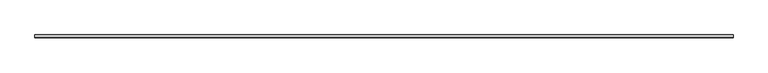
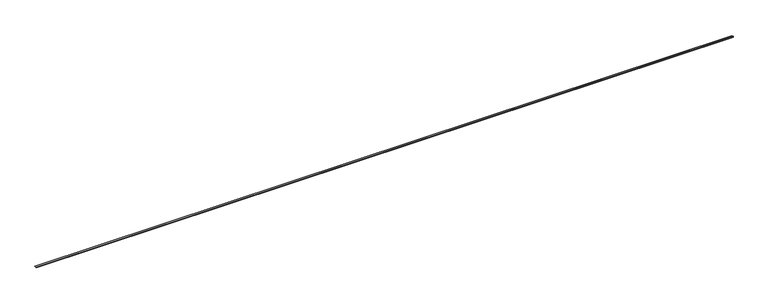
"""IFC4 building model written with IfcOpenShell, lengths in millimetres: proxy geometry, Generic Models 7:Generic Models 1:6:Generic Models 1:6 : Generic Models 7:Generic Models 1:337419:19 : Generic Models 7:Generic Models 1:6:Generic Models 1:6 : Generic Models 7:Generic Models 1:337419:312901."""

from ifc_helpers import new_model, si_unit, frame, origin, place, context, project, spatial, polyline, outline, extrude, source, transform, mapped, element, save


def generic_models_74043bfa(model_context):
    return source(origin(), model_context, "Body", "SweptSolid", [
        extrude(outline(polyline([(-578453.7976341, -216.69375), (-578453.7976341, -218.28125), (-578885.5976341, -218.28125), (-578885.5976341, -97.507466), (-578884.0101341, -97.507466), (-578884.0101341, -216.69375), (-578453.7976341, -216.69375)])), frame((557771.6867239, 0.0, 0.0), z_axis=(1.0, 0.0, 0.0), x_axis=(0.0, 1.0, 0.0)), (0.0, 0.0, 1.0), 109559.725),
    ])


if __name__ == "__main__":
    model = new_model("IFC4")
    model_context = context("Model", 3, world=origin())
    ifc_project = project(units=[si_unit("LENGTHUNIT", "METRE", prefix="MILLI")], contexts=[model_context])
    site = spatial("IfcSite", under=ifc_project)
    building = spatial("IfcBuilding", under=site)
    placement = place(None, origin())
    generic_models_shape = generic_models_74043bfa(model_context)
    element("IfcBuildingElementProxy", 1, Name="Generic Models 7:Generic Models 1:6:Generic Models 1:6 : Generic Models 7:Generic Models 1:337419:19 : Generic Models 7:Generic Models 1:6:Generic Models 1:6 : Generic Models 7:Generic Models 1:337419:312901", ObjectType="Generic Models 7:Generic Models 1:6:Generic Models 1:6 : Generic Models 7:Generic Models 1:337419:19 : Generic Models 7:Generic Models 1:6:Generic Models 1:6 : Generic Models 7:Generic Models 1:337419:312901", at=placement, inside=building, context=model_context, shape_type="MappedRepresentation", body=[
        mapped(generic_models_shape, transform((0.0, 0.0, 0.0), x_axis=(1.0, 0.0, 0.0), y_axis=(0.0, 1.0, 0.0), z_axis=(0.0, 0.0, 1.0))),
    ])
    save(model, "model.ifc")

# Revit data of these elements
# Type "Generic Models 7:Generic Models 1:6:Generic Models 1:6 : Generic Models 7:Generic Models 1:337419:19 : Generic Models 7:Generic Models 1:6:Generic Models 1:6 : Generic Models 7:Generic Models 1:337419:312901"
#   NameOverride = "Generic Models 7:Generic Models 1:6:Generic Models 1:6 : Generic Models 7:Generic Models 1:337419:312901"
#   ObjectTypeOverride = "Generic Models 1:6 : Generic Models 7:Generic Models 1:337419"
#   Reference = "Generic Models 1"
#   Tag = "312901"
# Element 1 (IfcBuildingElementProxy, "Generic Models 7:Generic Models 1:6:Generic Models 1:6 : Generic Models 7:Generic Models 1:337419:19 : Generic Models 7:Generic Models 1:6:Generic Models 1:6 : Generic Models 7:Generic Models 1:337419:312901")
#   Materials on its faces: "VAPOR BARRIER"
# Materials
#   "VAPOR BARRIER": class "Generic", colour RGB 66 158 52, transparency 0, Cost = 0
